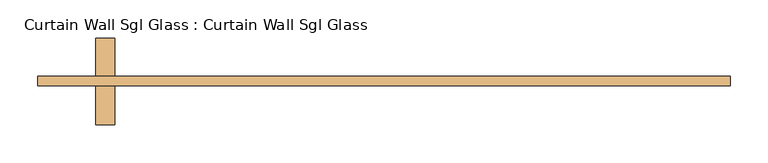
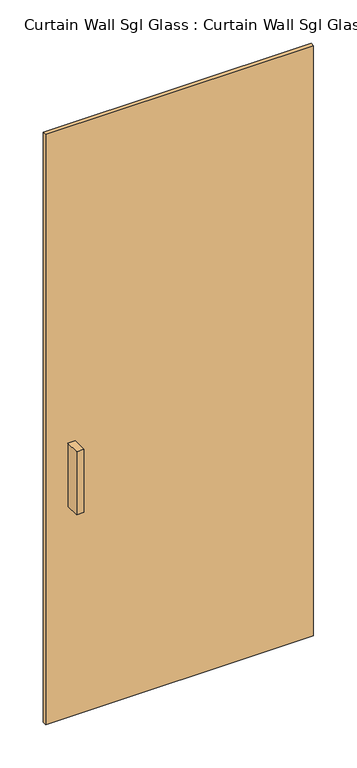
"""IFC4 building model written with IfcOpenShell, lengths in millimetres: door geometry, Curtain Wall Sgl Glass : Curtain Wall Sgl Glass."""

import ifcopenshell
import ifcopenshell.guid

model = None  # the IFC model being written
_history = None  # IfcOwnerHistory: only IFC2X3 demands one
_inside = {}  # id of a spatial element -> (the spatial element, [elements in it])
_under = {}  # id of a project, library or spatial element -> (it, [spatial elements below it])
_declared = {}  # id of a project -> (the project, [libraries it declares])
_typed = {}  # id of a type object -> (the type object, [elements of that type])
_made_of = {}  # id of a material, layer set ... -> (it, [elements and type objects made of it])


def new_model(schema):
    """Start an empty IFC model of exactly this schema.

    Asked for "IFC4X3", IfcOpenShell would pick the latest addendum, in which some entities
    have other attributes; the version numbers below select the first issue.
    IFC2X3 requires an IfcOwnerHistory on every rooted entity: one is made here for all.
    """
    global model, _history
    if schema == "IFC4X3":
        model = ifcopenshell.file(schema_version=(4, 3, 0, 0))
    else:
        model = ifcopenshell.file(schema=schema)
    _inside.clear()
    _under.clear()
    _declared.clear()
    _typed.clear()
    _made_of.clear()
    _history = None
    if model.schema == "IFC2X3":
        org = make("IfcOrganization", Name="unknown")
        user = make(
            "IfcPersonAndOrganization",
            ThePerson=make("IfcPerson", FamilyName="unknown"),
            TheOrganization=org,
        )
        app = make(
            "IfcApplication",
            ApplicationDeveloper=org,
            Version="unknown",
            ApplicationFullName="unknown",
            ApplicationIdentifier="unknown",
        )
        _history = make(
            "IfcOwnerHistory",
            OwningUser=user,
            OwningApplication=app,
            ChangeAction="ADDED",
            CreationDate=0,
        )
    return model


def make(cls, **values):
    """One entity of the class cls with the attributes given. An attribute that is None is left unset."""
    return model.create_entity(
        cls, **{name: value for name, value in values.items() if value is not None}
    )


def rooted(cls, **values):
    """An entity with a GlobalId (a new one), such as an element, a storey or a relation."""
    return make(cls, GlobalId=ifcopenshell.guid.new(), OwnerHistory=_history, **values)


def si_unit(unit_type, name, prefix=None):
    """IfcSIUnit, for example si_unit("LENGTHUNIT", "METRE", prefix="MILLI")."""
    return make("IfcSIUnit", UnitType=unit_type, Prefix=prefix, Name=name)


def assignment(units):
    """IfcUnitAssignment: the units of a project."""
    return None if units is None else make("IfcUnitAssignment", Units=units)


def point(xyz):
    """IfcCartesianPoint."""
    return None if xyz is None else make("IfcCartesianPoint", Coordinates=xyz)


def direction(xyz):
    """IfcDirection."""
    return None if xyz is None else make("IfcDirection", DirectionRatios=xyz)


def frame(location, z_axis=None, x_axis=None):
    """IfcAxis2Placement3D, a coordinate frame: its origin and axes. An axis left out is left unset."""
    return make(
        "IfcAxis2Placement3D",
        Location=point(location),
        Axis=direction(z_axis),
        RefDirection=direction(x_axis),
    )


def origin():
    """The frame at (0, 0, 0) with its axes left unset."""
    return frame((0.0, 0.0, 0.0))


def origin_with_axes():
    """The frame at (0, 0, 0) with the z axis (0, 0, 1) and the x axis (1, 0, 0) written out."""
    return frame((0.0, 0.0, 0.0), z_axis=(0.0, 0.0, 1.0), x_axis=(1.0, 0.0, 0.0))


def place(relative_to, where):
    """IfcLocalPlacement: puts the frame where relative to a parent placement (None: the world)."""
    return make(
        "IfcLocalPlacement", PlacementRelTo=relative_to, RelativePlacement=where
    )


def context(
    kind, dimensions, precision=None, world=None, true_north=None, identifier=None
):
    """IfcGeometricRepresentationContext, for example the 3D "Model" context."""
    return make(
        "IfcGeometricRepresentationContext",
        ContextIdentifier=identifier,
        ContextType=kind,
        CoordinateSpaceDimension=dimensions,
        Precision=precision,
        WorldCoordinateSystem=world,
        TrueNorth=true_north,
    )


def project(units=None, contexts=None):
    """IfcProject with its units and contexts."""
    return rooted(
        "IfcProject",
        Name="project",
        RepresentationContexts=contexts,
        UnitsInContext=assignment(units),
    )


def spatial(cls, under=None, at=None, **own):
    """A site, building, storey or space (cls), placed at a placement, below another one or the project."""
    s = rooted(cls, ObjectPlacement=at, **own)
    if under is not None:
        _under.setdefault(under.id(), (under, []))[1].append(s)
    return s


def polyline(points):
    """IfcPolyline through the points."""
    return make("IfcPolyline", Points=[point(p) for p in points])


def outline(outer, holes=None, kind="AREA"):
    """IfcArbitraryClosedProfileDef: a profile drawn as a closed curve; with holes, ...WithVoids."""
    if holes is None:
        return make("IfcArbitraryClosedProfileDef", ProfileType=kind, OuterCurve=outer)
    return make(
        "IfcArbitraryProfileDefWithVoids",
        ProfileType=kind,
        OuterCurve=outer,
        InnerCurves=holes,
    )


def extrude(swept, where, along, depth):
    """IfcExtrudedAreaSolid: the profile swept, set in the frame where, extruded along a direction by depth."""
    return make(
        "IfcExtrudedAreaSolid",
        SweptArea=swept,
        Position=where,
        ExtrudedDirection=direction(along),
        Depth=depth,
    )


def shape(context_of_items, identifier, shape_type, items):
    """IfcShapeRepresentation: the items that make up one representation, for example the "Body"."""
    return make(
        "IfcShapeRepresentation",
        ContextOfItems=context_of_items,
        RepresentationIdentifier=identifier,
        RepresentationType=shape_type,
        Items=items,
    )


def source(mapping_origin, context_of_items, identifier, shape_type, items):
    """IfcRepresentationMap: a shape defined once, which mapped items show again and again."""
    return make(
        "IfcRepresentationMap",
        MappingOrigin=mapping_origin,
        MappedRepresentation=shape(context_of_items, identifier, shape_type, items),
    )


def transform(
    local_origin,
    x_axis=None,
    y_axis=None,
    z_axis=None,
    scale=None,
    scale2=None,
    scale3=None,
    uniform=True,
):
    """IfcCartesianTransformationOperator3D, or its non-uniform kind. x_axis, y_axis, z_axis: its Axis1, 2, 3."""
    if uniform:
        return make(
            "IfcCartesianTransformationOperator3D",
            Axis1=direction(x_axis),
            Axis2=direction(y_axis),
            LocalOrigin=point(local_origin),
            Scale=scale,
            Axis3=direction(z_axis),
        )
    return make(
        "IfcCartesianTransformationOperator3DnonUniform",
        Axis1=direction(x_axis),
        Axis2=direction(y_axis),
        LocalOrigin=point(local_origin),
        Scale=scale,
        Axis3=direction(z_axis),
        Scale2=scale2,
        Scale3=scale3,
    )


def mapped(mapping_source, mapping_target):
    """IfcMappedItem: shows the shape of a source again, moved by a transform."""
    return make(
        "IfcMappedItem", MappingSource=mapping_source, MappingTarget=mapping_target
    )


def made_of(thing, what):
    """Note that an element or type object is made of a material, layer set ...; save() writes the relation."""
    if what is not None:
        _made_of.setdefault(what.id(), (what, []))[1].append(thing)
    return thing


def element(
    cls,
    number,
    at=None,
    inside=None,
    cuts=None,
    type_object=None,
    material=None,
    context=None,
    identifier="Body",
    shape_type=None,
    held_by="IfcProductDefinitionShape",
    body=None,
    shapes=None,
    **own,
):
    """One element of the class cls, such as IfcWall. Its Tag is "e" and its number.

    at: its placement. inside: the storey or other place that contains it. cuts: it is an
    opening in that element (IfcRelVoidsElement). A single representation is given by context,
    identifier, shape_type and body (its items); several are given by shapes. held_by: the class
    of the entity that holds the representations. save() writes the other relations.
    """
    e = rooted(cls, Tag="e%d" % number, ObjectPlacement=at, **own)
    if body is not None:
        shapes = [shape(context, identifier, shape_type, body)]
    if shapes is not None:
        e.Representation = make(held_by, Representations=shapes)
    if inside is not None:
        _inside.setdefault(inside.id(), (inside, []))[1].append(e)
    if cuts is not None:
        rooted(
            "IfcRelVoidsElement", RelatingBuildingElement=cuts, RelatedOpeningElement=e
        )
    if type_object is not None:
        _typed.setdefault(type_object.id(), (type_object, []))[1].append(e)
    return made_of(e, material)


def aggregate(whole, parts):
    """IfcRelAggregates: a whole, such as a stair, and the parts it consists of."""
    return rooted("IfcRelAggregates", RelatingObject=whole, RelatedObjects=parts)


def save(model, path):
    """Write the relations noted so far, then the file.

    IfcRelAggregates (storeys below a building ...), IfcRelContainedInSpatialStructure (elements
    in a storey), IfcRelDefinesByType, IfcRelAssociatesMaterial and IfcRelDeclares: one each for
    every whole, place, type object, material and project.
    """
    for whole, parts in _under.values():
        aggregate(whole, parts)
    for where, things in _inside.values():
        rooted(
            "IfcRelContainedInSpatialStructure",
            RelatedElements=things,
            RelatingStructure=where,
        )
    for kind, things in _typed.values():
        rooted("IfcRelDefinesByType", RelatedObjects=things, RelatingType=kind)
    for what, things in _made_of.values():
        rooted("IfcRelAssociatesMaterial", RelatedObjects=things, RelatingMaterial=what)
    for by, libraries in _declared.values():
        rooted("IfcRelDeclares", RelatingContext=by, RelatedDefinitions=libraries)
    model.write(path)


def curtain_wall_sgl_glass_curtain_wall_sgl_glass_c2d4b377(model_context):
    return source(origin(), model_context, "Body", "SweptSolid", [
        extrude(outline(polyline([(-355.6, 12.7), (-355.6, -38.1), (-381.0, -38.1), (-381.0, 12.7), (-355.6, 12.7)])), frame((0.0, 0.0, 762.0), z_axis=(0.0, 0.0, 1.0), x_axis=(1.0, 0.0, 0.0)), (0.0, 0.0, 1.0), 228.6),
        extrude(outline(polyline([(-381.0, -101.6), (-381.0, -50.8), (-355.6, -50.8), (-355.6, -101.6), (-381.0, -101.6)])), frame((0.0, 0.0, 762.0), z_axis=(0.0, 0.0, 1.0), x_axis=(1.0, 0.0, 0.0)), (0.0, 0.0, 1.0), 228.6),
        extrude(outline(polyline([(457.2, -50.8), (-457.2, -50.8), (-457.2, -38.1), (457.2, -38.1), (457.2, -50.8)])), origin_with_axes(), (0.0, 0.0, 1.0), 2133.6),
    ])


if __name__ == "__main__":
    model = new_model("IFC4")
    model_context = context("Model", 3, world=origin())
    ifc_project = project(units=[si_unit("LENGTHUNIT", "METRE", prefix="MILLI")], contexts=[model_context])
    site = spatial("IfcSite", under=ifc_project)
    building = spatial("IfcBuilding", under=site)
    placement = place(None, origin())
    curtain_wall_sgl_glass_curtain_wall_sgl_glass_shape = curtain_wall_sgl_glass_curtain_wall_sgl_glass_c2d4b377(model_context)
    element("IfcDoor", 1, ObjectType="Curtain Wall Sgl Glass : Curtain Wall Sgl Glass", at=placement, inside=building, context=model_context, shape_type="MappedRepresentation", body=[
        mapped(curtain_wall_sgl_glass_curtain_wall_sgl_glass_shape, transform((0.0, 0.0, 0.0), x_axis=(1.0, 0.0, 0.0), y_axis=(0.0, 1.0, 0.0), z_axis=(0.0, 0.0, 1.0))),
    ])
    save(model, "model.ifc")

# Revit data of these elements
# Type "Curtain Wall Sgl Glass : Curtain Wall Sgl Glass"
#   Assembly Code = "B2030100"
#   Offset = 0' - 2"
#   Function = 1
#   Handle Material = Metal - Aluminum
#   Glazing Material = Glass
# Element 1 (IfcDoor, "Curtain Wall Sgl Glass : Curtain Wall Sgl Glass")
#   Materials on its faces: "Metal - Aluminum", "Glass"
# Materials
#   "Metal - Aluminum": class "Metal", colour RGB 140 140 140, transparency 0
#   "Glass": class "Glass", colour RGB 0 128 192, transparency 0.75
